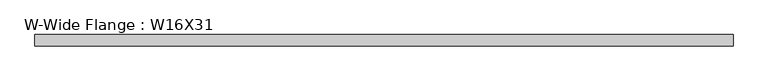
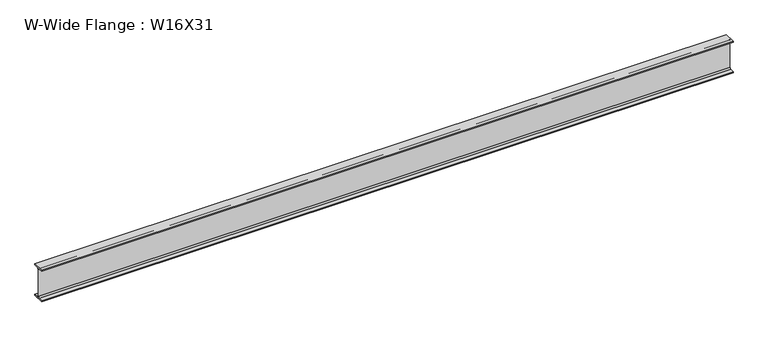
"""IFC4 building model written with IfcOpenShell, lengths in millimetres: beam geometry, W-Wide Flange : W16X31."""

from ifc_helpers import new_model, si_unit, point, frame, frame_2d, origin, place, context, project, spatial, polyline, circle_curve, trimmed, segment, composite_curve, outline, extrude, source, transform, mapped, element, save


def w_wide_flange_w16x31_951fd6ce(model_context):
    return source(origin(), model_context, "Body", "SweptSolid", [
        extrude(outline(composite_curve([segment(polyline([(70.231, -190.754), (70.231, -201.93), (-70.231, -201.93), (-70.231, -190.754), (-20.8915, -190.754)]), True, "CONTINUOUS"), segment(trimmed(circle_curve(frame_2d((-20.8915, -173.355)), 17.399), [point((-20.8915, -190.754))], [point((-3.4925, -173.355))], True, "CARTESIAN"), True, "CONTINUOUS"), segment(polyline([(-3.4925, -173.355), (-3.4925, 173.355)]), True, "CONTINUOUS"), segment(trimmed(circle_curve(frame_2d((-20.8915, 173.355)), 17.399), [point((-3.4925, 173.355))], [point((-20.8915, 190.754))], True, "CARTESIAN"), True, "CONTINUOUS"), segment(polyline([(-20.8915, 190.754), (-70.231, 190.754), (-70.231, 201.93), (70.231, 201.93), (70.231, 190.754), (20.8915, 190.754)]), True, "CONTINUOUS"), segment(trimmed(circle_curve(frame_2d((20.8915, 173.355)), 17.399), [point((20.8915, 190.754))], [point((3.4925, 173.355))], True, "CARTESIAN"), True, "CONTINUOUS"), segment(polyline([(3.4925, 173.355), (3.4925, -173.355)]), True, "CONTINUOUS"), segment(trimmed(circle_curve(frame_2d((20.8915, -173.355)), 17.399), [point((3.4925, -173.355))], [point((20.8915, -190.754))], True, "CARTESIAN"), True, "CONTINUOUS"), segment(polyline([(20.8915, -190.754), (70.231, -190.754)]), True, "CONTINUOUS")], self_intersect=False)), frame((-4221.9066406, 0.0, 0.0), z_axis=(1.0, 0.0, 0.0), x_axis=(0.0, 1.0, 0.0)), (0.0, 0.0, 1.0), 8493.8195313),
    ])


if __name__ == "__main__":
    model = new_model("IFC4")
    model_context = context("Model", 3, world=origin())
    ifc_project = project(units=[si_unit("LENGTHUNIT", "METRE", prefix="MILLI")], contexts=[model_context])
    site = spatial("IfcSite", under=ifc_project)
    building = spatial("IfcBuilding", under=site)
    placement = place(None, origin())
    w_wide_flange_w16x31_shape = w_wide_flange_w16x31_951fd6ce(model_context)
    element("IfcBeam", 1, ObjectType="W-Wide Flange : W16X31", at=placement, inside=building, context=model_context, shape_type="MappedRepresentation", body=[
        mapped(w_wide_flange_w16x31_shape, transform((0.0, 0.0, 0.0), x_axis=(1.0, 0.0, 0.0), y_axis=(0.0, 1.0, 0.0), z_axis=(0.0, 0.0, 1.0))),
    ])
    save(model, "model.ifc")

# Revit data of these elements
# Type "W-Wide Flange : W16X31"
#   Assembly Code = "B10"
#   W = 31
#   Length [instance default] = 1524 mm
#   bf = 140.462 mm
#   d = 403.86 mm
#   k = 28.575 mm
#   k2 = 17.399 mm
#   tf = 11.176 mm
#   tw = 6.985 mm
#   A = 0.00589031 m²
#   Structural Material [instance default] = Steel ASTM A992
# Element 1 (IfcBeam, "W-Wide Flange : W16X31")
#   Structural Material = Aluminum, Anodized Red
#   Materials on its faces: "Aluminum, Anodized Red"
# Materials
#   "Steel ASTM A992": class "Metal", colour RGB 128 0 0, transparency 0, Description = "Structural steel 50ksi", Cost = 0
#   "Aluminum, Anodized Red": class "Metal", colour RGB 120 120 120, transparency 0, Description = "Anodized aluminum, red", Cost = 0
